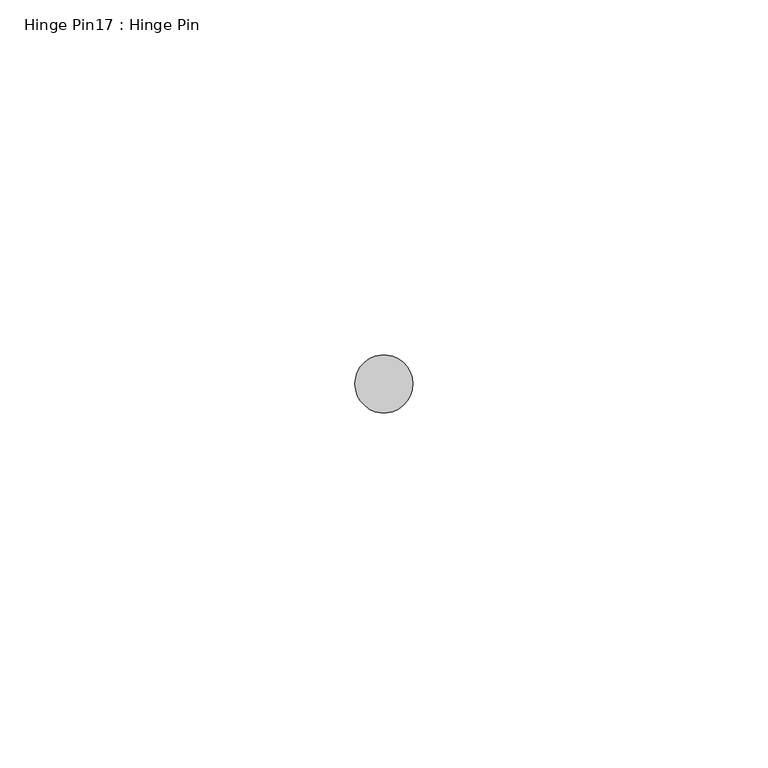
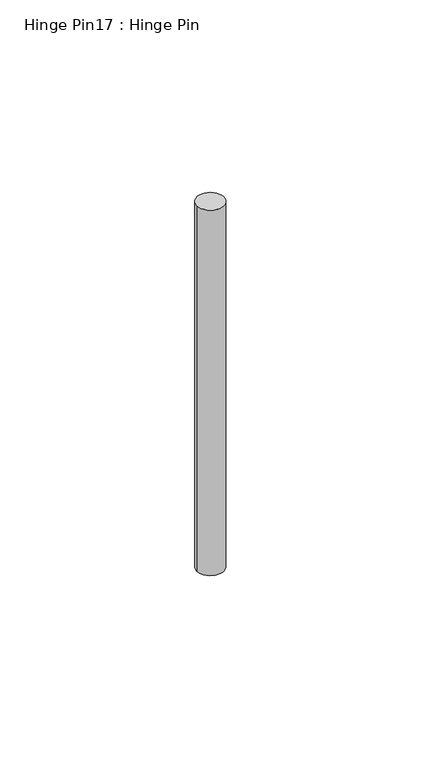
"""IFC4 building model written with IfcOpenShell, lengths in millimetres: proxy geometry, Hinge Pin17 : Hinge Pin."""

from ifc_helpers import new_model, si_unit, point, frame, frame_2d, origin, place, context, project, spatial, circle_curve, trimmed, segment, composite_curve, outline, extrude, source, transform, mapped, element, save


def hinge_pin17_hinge_pin_e8284dc3(model_context):
    return source(origin(), model_context, "Body", "SweptSolid", [
        extrude(outline(composite_curve([segment(trimmed(circle_curve(frame_2d((587319.1320739, -533984.6777841)), 4.0894), [point((587315.0426739, -533984.6777841))], [point((587323.2214739, -533984.6777841))], False, "CARTESIAN"), True, "CONTINUOUS"), segment(trimmed(circle_curve(frame_2d((587319.1320739, -533984.6777841)), 4.0894), [point((587323.2214739, -533984.6777841))], [point((587315.0426739, -533984.6777841))], False, "CARTESIAN"), True, "CONTINUOUS")], self_intersect=False)), frame((0.0, 0.0, 1128.5140625), z_axis=(0.0, 0.0, 1.0), x_axis=(1.0, 0.0, 0.0)), (0.0, 0.0, 1.0), 117.871875),
    ])


if __name__ == "__main__":
    model = new_model("IFC4")
    model_context = context("Model", 3, world=origin())
    ifc_project = project(units=[si_unit("LENGTHUNIT", "METRE", prefix="MILLI")], contexts=[model_context])
    site = spatial("IfcSite", under=ifc_project)
    building = spatial("IfcBuilding", under=site)
    placement = place(None, origin())
    hinge_pin17_hinge_pin_shape = hinge_pin17_hinge_pin_e8284dc3(model_context)
    element("IfcBuildingElementProxy", 1, Name="Hinge Pin17 : Hinge Pin", ObjectType="Hinge Pin17 : Hinge Pin", at=placement, inside=building, context=model_context, shape_type="MappedRepresentation", body=[
        mapped(hinge_pin17_hinge_pin_shape, transform((0.0, 0.0, 0.0), x_axis=(1.0, 0.0, 0.0), y_axis=(0.0, 1.0, 0.0), z_axis=(0.0, 0.0, 1.0))),
    ])
    save(model, "model.ifc")

# Revit data of these elements
# Element 1 (IfcBuildingElementProxy, "Hinge Pin17 : Hinge Pin")
#   Materials on its faces: "6\"X6\" WELD-ON STL BUTT HINGE"
# Materials
#   "6\"X6\" WELD-ON STL BUTT HINGE": class "Metal", colour RGB 189 187 185, transparency 0, Description = "Carbon steel", Cost = 0
